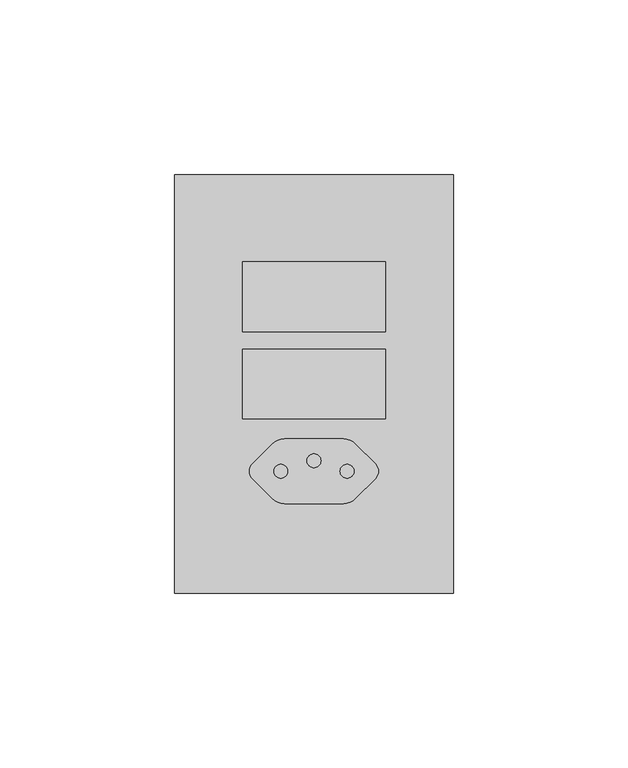
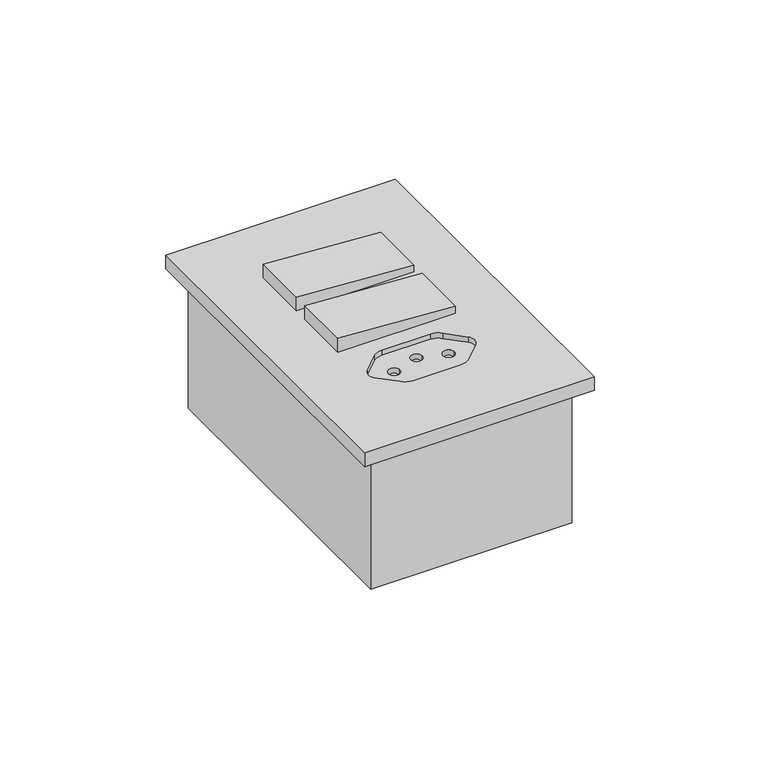
"""IFC4 building model written with IfcOpenShell, lengths in millimetres: proxy geometry, CAIXA VERTICE V7 : Interruptor 2s + Tomada 10A 1s."""

from ifc_helpers import new_model, si_unit, frame, origin, place, context, project, spatial, polyline, circle_curve, outline, extrude, faceted_brep, source, transform, mapped, element, save
from ifc_brep_helpers import plane_surface, revolved_surface, advanced_brep


def electrical_fixtures_1a926fea(model_context):
    return source(origin(), model_context, "Body", "SolidModel", [
        extrude(outline(polyline([(5.0, 20.5), (7.5, 20.5), (10.0, -20.5), (5.0, -20.5), (5.0, 20.5)])), frame((0.0, 1090.0, 0.0), z_axis=(0.0, 1.0, 0.0), x_axis=(0.0, 0.0, 1.0)), (0.0, 0.0, 1.0), 20.0),
        extrude(outline(polyline([(5.0, 20.5), (7.5, 20.5), (10.0, -20.5), (5.0, -20.5), (5.0, 20.5)])), frame((0.0, 1115.0, 0.0), z_axis=(0.0, 1.0, 0.0), x_axis=(0.0, 0.0, 1.0)), (0.0, 0.0, 1.0), 20.0),
        faceted_brep([(33.0, 1047.0, -48.0), (33.0, 1153.0, -48.0), (-33.0, 1153.0, -48.0), (-33.0, 1047.0, -48.0), (35.0, 1155.0, -50.0), (35.0, 1045.0, -50.0), (-35.0, 1045.0, -50.0), (-35.0, 1155.0, -50.0), (-35.0, 1155.0, 0.0), (35.0, 1155.0, 0.0), (-35.0, 1045.0, 0.0), (35.0, 1045.0, 0.0), (33.0, 1153.0, 0.0), (33.0, 1047.0, 0.0), (-33.0, 1047.0, 0.0), (-33.0, 1153.0, 0.0)], [[[0, 1, 2, 3]], [[4, 5, 6, 7]], [[4, 7, 8, 9]], [[8, 7, 6, 10]], [[10, 6, 5, 11]], [[11, 5, 4, 9]], [[9, 8, 10, 11], [12, 13, 14, 15]], [[13, 12, 1, 0]], [[14, 13, 0, 3]], [[15, 14, 3, 2]], [[12, 15, 2, 1]]]),
        advanced_brep(
        [(40.0, 1160.0, 5.0), (-40.0, 1160.0, 5.0), (-40.0, 1040.0, 5.0), (40.0, 1040.0, 5.0), (8.4215729, 1065.75, 5.0), (-8.4215729, 1065.75, 5.0), (-11.9571068, 1067.2144661, 5.0), (-17.6213203, 1072.8786797, 5.0), (-17.6213203, 1077.1213203, 5.0), (-11.9571068, 1082.7855339, 5.0), (-8.4215729, 1084.25, 5.0), (8.4215729, 1084.25, 5.0), (11.9571068, 1082.7855339, 5.0), (17.6213203, 1077.1213203, 5.0), (17.6213203, 1072.8786797, 5.0), (11.9571068, 1067.2144661, 5.0), (-40.0, 1160.0, 0.0), (40.0, 1160.0, 0.0), (40.0, 1040.0, 0.0), (-40.0, 1040.0, 0.0), (8.4215729, 1065.75, 3.0), (11.9571068, 1067.2144661, 3.0), (17.6213203, 1072.8786797, 3.0), (17.6213203, 1077.1213203, 3.0), (11.9571068, 1082.7855339, 3.0), (8.4215729, 1084.25, 3.0), (-8.4215729, 1084.25, 3.0), (-11.9571068, 1082.7855339, 3.0), (-17.6213203, 1077.1213203, 3.0), (-17.6213203, 1072.8786797, 3.0), (-11.9571068, 1067.2144661, 3.0), (-8.4215729, 1065.75, 3.0), (-7.5, 1075.0, 3.0), (-11.5, 1075.0, 3.0), (11.5, 1075.0, 3.0), (7.5, 1075.0, 3.0), (2.0, 1078.0, 3.0), (-2.0, 1078.0, 3.0), (-11.5, 1075.0, 1.0), (-7.5, 1075.0, 1.0), (7.5, 1075.0, 1.0), (11.5, 1075.0, 1.0), (-2.0, 1078.0, 1.0), (2.0, 1078.0, 1.0)],
        [
            (0, 1),
            (1, 2),
            (2, 3),
            (3, 0),
            (4, 5),
            (5, 6, circle_curve(frame((-8.4215729, 1070.75, 5.0), z_axis=(0.0, 0.0, -1.0), x_axis=(-1.0, 0.0, 0.0)), 5.0)),
            (6, 7),
            (7, 8, circle_curve(frame((-15.5, 1075.0, 5.0), z_axis=(0.0, 0.0, -1.0), x_axis=(-1.0, 0.0, 0.0)), 3.0)),
            (8, 9),
            (9, 10, circle_curve(frame((-8.4215729, 1079.25, 5.0), z_axis=(0.0, 0.0, -1.0), x_axis=(-1.0, 0.0, 0.0)), 5.0)),
            (10, 11),
            (11, 12, circle_curve(frame((8.4215729, 1079.25, 5.0), z_axis=(0.0, 0.0, -1.0), x_axis=(-1.0, 0.0, 0.0)), 5.0)),
            (12, 13),
            (13, 14, circle_curve(frame((15.5, 1075.0, 5.0), z_axis=(0.0, 0.0, -1.0), x_axis=(-1.0, 0.0, 0.0)), 3.0)),
            (14, 15),
            (15, 4, circle_curve(frame((8.4215729, 1070.75, 5.0), z_axis=(0.0, 0.0, -1.0), x_axis=(-1.0, 0.0, 0.0)), 5.0)),
            (16, 17),
            (17, 18),
            (18, 19),
            (19, 16),
            (0, 17),
            (16, 1),
            (19, 2),
            (18, 3),
            (20, 21, circle_curve(frame((8.4215729, 1070.75, 3.0), z_axis=(0.0, 0.0, 1.0), x_axis=(-1.0, 0.0, 0.0)), 5.0)),
            (21, 22),
            (22, 23, circle_curve(frame((15.5, 1075.0, 3.0), z_axis=(0.0, 0.0, 1.0), x_axis=(-1.0, 0.0, 0.0)), 3.0)),
            (23, 24),
            (24, 25, circle_curve(frame((8.4215729, 1079.25, 3.0), z_axis=(0.0, 0.0, 1.0), x_axis=(-1.0, 0.0, 0.0)), 5.0)),
            (25, 26),
            (26, 27, circle_curve(frame((-8.4215729, 1079.25, 3.0), z_axis=(0.0, 0.0, 1.0), x_axis=(-1.0, 0.0, 0.0)), 5.0)),
            (27, 28),
            (28, 29, circle_curve(frame((-15.5, 1075.0, 3.0), z_axis=(0.0, 0.0, 1.0), x_axis=(-1.0, 0.0, 0.0)), 3.0)),
            (29, 30),
            (30, 31, circle_curve(frame((-8.4215729, 1070.75, 3.0), z_axis=(0.0, 0.0, 1.0), x_axis=(-1.0, 0.0, 0.0)), 5.0)),
            (31, 20),
            (32, 33, circle_curve(frame((-9.5, 1075.0, 3.0), z_axis=(0.0, 0.0, -1.0), x_axis=(1.0, 2.301812013077709e-12, 0.0)), 2.0)),
            (33, 32, circle_curve(frame((-9.5, 1075.0, 3.0), z_axis=(0.0, 0.0, -1.0), x_axis=(1.0, 2.301812013077709e-12, 0.0)), 2.0)),
            (34, 35, circle_curve(frame((9.5, 1075.0, 3.0), z_axis=(0.0, 0.0, -1.0), x_axis=(1.0, 2.301812013077709e-12, 0.0)), 2.0)),
            (35, 34, circle_curve(frame((9.5, 1075.0, 3.0), z_axis=(0.0, 0.0, -1.0), x_axis=(1.0, 2.301812013077709e-12, 0.0)), 2.0)),
            (36, 37, circle_curve(frame((0.0, 1078.0, 3.0), z_axis=(0.0, 0.0, -1.0), x_axis=(1.0, 2.301812013077709e-12, 0.0)), 2.0)),
            (37, 36, circle_curve(frame((0.0, 1078.0, 3.0), z_axis=(0.0, 0.0, -1.0), x_axis=(1.0, 2.301812013077709e-12, 0.0)), 2.0)),
            (31, 5),
            (4, 20),
            (30, 6),
            (29, 7),
            (28, 8),
            (27, 9),
            (26, 10),
            (25, 11),
            (24, 12),
            (23, 13),
            (22, 14),
            (21, 15),
            (38, 39, circle_curve(frame((-9.5, 1075.0, 1.0), z_axis=(0.0, 0.0, 1.0), x_axis=(1.0, 2.301812013077709e-12, 0.0)), 2.0)),
            (39, 38, circle_curve(frame((-9.5, 1075.0, 1.0), z_axis=(0.0, 0.0, 1.0), x_axis=(1.0, 2.301812013077709e-12, 0.0)), 2.0)),
            (40, 41, circle_curve(frame((9.5, 1075.0, 1.0), z_axis=(0.0, 0.0, 1.0), x_axis=(1.0, 2.301812013077709e-12, 0.0)), 2.0)),
            (41, 40, circle_curve(frame((9.5, 1075.0, 1.0), z_axis=(0.0, 0.0, 1.0), x_axis=(1.0, 2.301812013077709e-12, 0.0)), 2.0)),
            (42, 43, circle_curve(frame((0.0, 1078.0, 1.0), z_axis=(0.0, 0.0, 1.0), x_axis=(1.0, 2.301812013077709e-12, 0.0)), 2.0)),
            (43, 42, circle_curve(frame((0.0, 1078.0, 1.0), z_axis=(0.0, 0.0, 1.0), x_axis=(1.0, 2.301812013077709e-12, 0.0)), 2.0)),
            (32, 39),
            (38, 33),
            (34, 41),
            (40, 35),
            (36, 43),
            (42, 37),
        ],
        [
            plane_surface(frame((-60.0, 1160.0, 5.0), z_axis=(0.0, 0.0, 1.0), x_axis=(-1.0, 0.0, 0.0))),
            plane_surface(frame((-60.0, 1160.0, 0.0), z_axis=(0.0, 0.0, -1.0), x_axis=(1.0, 0.0, 0.0))),
            plane_surface(frame((40.0, 1160.0, 5.0), z_axis=(0.0, 1.0, 0.0), x_axis=(0.0, 0.0, -1.0))),
            plane_surface(frame((-40.0, 1160.0, 5.0), z_axis=(-1.0, 0.0, 0.0), x_axis=(0.0, 0.0, -1.0))),
            plane_surface(frame((-40.0, 1040.0, 5.0), z_axis=(0.0, -1.0, 0.0), x_axis=(0.0, 0.0, -1.0))),
            plane_surface(frame((40.0, 1040.0, 5.0), z_axis=(1.0, 0.0, 0.0), x_axis=(0.0, 0.0, -1.0))),
            plane_surface(frame((3.4215729, 1070.75, 3.0), z_axis=(0.0, 0.0, 1.0), x_axis=(0.0, 1.0, 0.0))),
            plane_surface(frame((-8.4215729, 1065.75, 5.0), z_axis=(0.0, 1.0, 0.0), x_axis=(0.0, 0.0, -1.0))),
            revolved_surface(polyline([(-13.4215729, 1070.75, 5.0), (-13.4215729, 1070.75, 3.0)]), (-8.4215729, 1070.75, 3.0), (0.0, 0.0, 1.0)),
            plane_surface(frame((-17.6213203, 1072.8786797, 5.0), z_axis=(0.7071067811865045, 0.7071067811865905, 0.0), x_axis=(0.0, 0.0, -1.0))),
            revolved_surface(polyline([(-18.5, 1075.0, 5.0), (-18.5, 1075.0, 3.0)]), (-15.5, 1075.0, 3.0), (0.0, 0.0, 1.0)),
            plane_surface(frame((-11.9571068, 1082.7855339, 5.0), z_axis=(0.7071067811865515, -0.7071067811865437, 0.0), x_axis=(0.0, 0.0, -1.0))),
            revolved_surface(polyline([(-13.4215729, 1079.25, 5.0), (-13.4215729, 1079.25, 3.0)]), (-8.4215729, 1079.25, 3.0), (0.0, 0.0, 1.0)),
            plane_surface(frame((8.4215729, 1084.25, 5.0), z_axis=(0.0, -1.0, 0.0), x_axis=(0.0, 0.0, -1.0))),
            revolved_surface(polyline([(3.4215728999999993, 1079.25, 5.0), (3.4215728999999993, 1079.25, 3.0)]), (8.4215729, 1079.25, 3.0), (0.0, 0.0, 1.0)),
            plane_surface(frame((17.6213203, 1077.1213203, 5.0), z_axis=(-0.7071067811865307, -0.7071067811865643, 0.0), x_axis=(0.0, 0.0, -1.0))),
            revolved_surface(polyline([(12.5, 1075.0, 5.0), (12.5, 1075.0, 3.0)]), (15.5, 1075.0, 3.0), (0.0, 0.0, 1.0)),
            plane_surface(frame((11.9571068, 1067.2144661, 5.0), z_axis=(-0.7071067811865893, 0.7071067811865058, 0.0), x_axis=(0.0, 0.0, -1.0))),
            revolved_surface(polyline([(3.4215728999999993, 1070.75, 5.0), (3.4215728999999993, 1070.75, 3.0)]), (8.4215729, 1070.75, 3.0), (0.0, 0.0, 1.0)),
            plane_surface(frame((-7.5, 1075.0, 1.0), z_axis=(0.0, 0.0, 1.0), x_axis=(2.301812013077709e-12, -1.0, 0.0))),
            revolved_surface(polyline([(-7.5, 1075.0000000000045, 3.0), (-7.5, 1075.0000000000045, 1.0)]), (-9.5, 1075.0, 1.0), (0.0, 0.0, 1.0)),
            revolved_surface(polyline([(11.5, 1075.0000000000045, 3.0), (11.5, 1075.0000000000045, 1.0)]), (9.5, 1075.0, 5.0), (0.0, 0.0, 1.0)),
            revolved_surface(polyline([(2.0, 1078.0000000000045, 3.0), (2.0, 1078.0000000000045, 1.0)]), (0.0, 1078.0, 5.0), (0.0, 0.0, 1.0)),
        ],
        [
            (0, [[1, 2, 3, 4], [5, 6, 7, 8, 9, 10, 11, 12, 13, 14, 15, 16]]),
            (1, [[17, 18, 19, 20]]),
            (2, [[-1, 21, -17, 22]]),
            (3, [[-2, -22, -20, 23]]),
            (4, [[-3, -23, -19, 24]]),
            (5, [[-4, -24, -18, -21]]),
            (6, [[25, 26, 27, 28, 29, 30, 31, 32, 33, 34, 35, 36], [37, 38], [39, 40], [41, 42]]),
            (7, [[-36, 43, -5, 44]]),
            (8, [[-35, 45, -6, -43]]),
            (9, [[-34, 46, -7, -45]]),
            (10, [[-33, 47, -8, -46]]),
            (11, [[-32, 48, -9, -47]]),
            (12, [[-31, 49, -10, -48]]),
            (13, [[-30, 50, -11, -49]]),
            (14, [[-29, 51, -12, -50]]),
            (15, [[-28, 52, -13, -51]]),
            (16, [[-27, 53, -14, -52]]),
            (17, [[-26, 54, -15, -53]]),
            (18, [[-25, -44, -16, -54]]),
            (19, [[55, 56]]),
            (19, [[57, 58]]),
            (19, [[59, 60]]),
            (20, [[-37, 61, -55, 62]]),
            (20, [[-38, -62, -56, -61]]),
            (21, [[-39, 63, -57, 64]]),
            (21, [[-40, -64, -58, -63]]),
            (22, [[-41, 65, -59, 66]]),
            (22, [[-42, -66, -60, -65]]),
        ],
    ),
    ])


if __name__ == "__main__":
    model = new_model("IFC4")
    model_context = context("Model", 3, world=origin())
    ifc_project = project(units=[si_unit("LENGTHUNIT", "METRE", prefix="MILLI")], contexts=[model_context])
    site = spatial("IfcSite", under=ifc_project)
    building = spatial("IfcBuilding", under=site)
    placement = place(None, origin())
    electrical_fixtures_shape = electrical_fixtures_1a926fea(model_context)
    element("IfcBuildingElementProxy", 1, Name="CAIXA VERTICE V7 : Interruptor 2s + Tomada 10A 1s", ObjectType="CAIXA VERTICE V7 : Interruptor 2s + Tomada 10A 1s", at=placement, inside=building, context=model_context, shape_type="MappedRepresentation", body=[
        mapped(electrical_fixtures_shape, transform((0.0, 0.0, 0.0), x_axis=(1.0, 0.0, 0.0), y_axis=(0.0, 1.0, 0.0), z_axis=(0.0, 0.0, 1.0))),
    ])
    save(model, "model.ifc")

# Revit data of these elements
# Type "CAIXA VERTICE V7 : Interruptor 2s + Tomada 10A 1s"
#   URL = "www.facebook.com/verticetreinamentos"
#   SEÇÃO [instance default] = ""
#   Rotação [instance default] = 0.00°
#   LARGURA DA TAMPA = 0.08 m
#   BORDA = 0.01 m
#   ALTURA DE INSTALAÇÃO [instance default] = 1.10 m
#   Distância Anotação [instance default] = 0.0015 m
#   ALTURA DA TAMPA = 0.12 m
#   Vertical [instance default] = yes
#   VER SEÇÃO [instance default] = yes
#   SHADE ESQ [instance default] = no
#   SHADE DIR [instance default] = yes
#   HORIZONTAL [instance default] = no
#   ANDAR COM A LEGENDA [instance default] = 0
#   Material Tampa [instance default] = Plástico, branco opaco
#   Caixa = element 1798552
#   Anotação = element 1798540
#   Default Elevation = 0
# Element 1 (IfcBuildingElementProxy, "CAIXA VERTICE V7 : Interruptor 2s + Tomada 10A 1s")
#   SEÇÃO = "2"
#   Materials on its faces: "Plástico, branco opaco"
# Materials
#   "Plástico, branco opaco": class "Plástico", colour RGB 120 120 120, transparency 0, Description = "Plastic, generic, opaque white", Cost = 0
